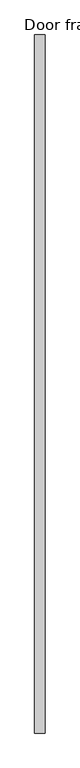
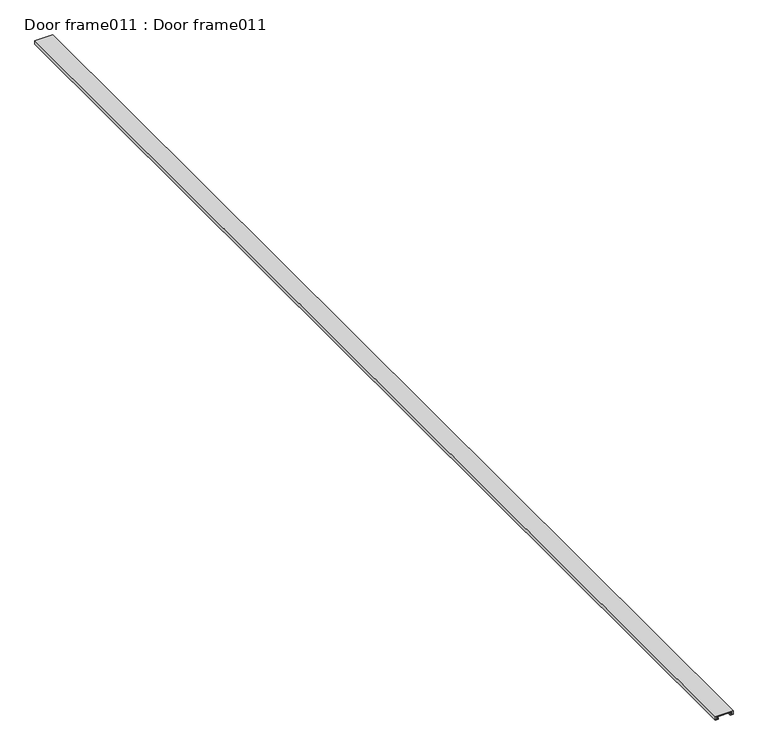
"""IFC4 building model written with IfcOpenShell, lengths in millimetres: proxy geometry, Door frame011 : Door frame011."""

from ifc_helpers import new_model, si_unit, frame, origin, place, context, project, spatial, polyline, outline, extrude, source, transform, mapped, element, save


def door_frame011_door_frame011_5bdfa61c(model_context):
    return source(origin(), model_context, "Body", "SweptSolid", [
        extrude(outline(polyline([(36591.6240434, 15510.0170405), (36585.6418094, 15510.0170405), (36585.6418094, 15514.9588645), (36588.2201312, 15514.9588645), (36588.2201312, 15513.9184805), (36586.9422894, 15513.9184805), (36586.9422894, 15511.3174945), (36590.0634674, 15511.3174945), (36590.0634674, 15538.9397417), (36586.9422894, 15538.9397417), (36586.9422894, 15536.538273), (36588.2201312, 15536.538273), (36588.2201312, 15535.2983717), (36585.6418094, 15535.2983717), (36585.6418094, 15540.2401957), (36591.6240434, 15540.2401957), (36591.6240434, 15510.0170405)])), frame((0.0, -1052.8906567, 0.0), z_axis=(0.0, 1.0, 0.0), x_axis=(0.0, 0.0, 1.0)), (0.0, 0.0, 1.0), 1999.85),
    ])


if __name__ == "__main__":
    model = new_model("IFC4")
    model_context = context("Model", 3, world=origin())
    ifc_project = project(units=[si_unit("LENGTHUNIT", "METRE", prefix="MILLI")], contexts=[model_context])
    site = spatial("IfcSite", under=ifc_project)
    building = spatial("IfcBuilding", under=site)
    placement = place(None, origin())
    door_frame011_door_frame011_shape = door_frame011_door_frame011_5bdfa61c(model_context)
    element("IfcBuildingElementProxy", 1, Name="Door frame011 : Door frame011", ObjectType="Door frame011 : Door frame011", at=placement, inside=building, context=model_context, shape_type="MappedRepresentation", body=[
        mapped(door_frame011_door_frame011_shape, transform((0.0, 0.0, 0.0), x_axis=(1.0, 0.0, 0.0), y_axis=(0.0, 1.0, 0.0), z_axis=(0.0, 0.0, 1.0))),
    ])
    save(model, "model.ifc")

# Revit data of these elements
# Type "Door frame011 : Door frame011"
#   NameOverride = "Door frame011"
# Element 1 (IfcBuildingElementProxy, "Door frame011 : Door frame011")
#   Materials on its faces: "FLEETWOOD SERIES T-3200 SINGLE SWING DOOR FRAME"
# Materials
#   "FLEETWOOD SERIES T-3200 SINGLE SWING DOOR FRAME": class "Unassigned", colour RGB 128 128 128, transparency 0, Cost = 0
